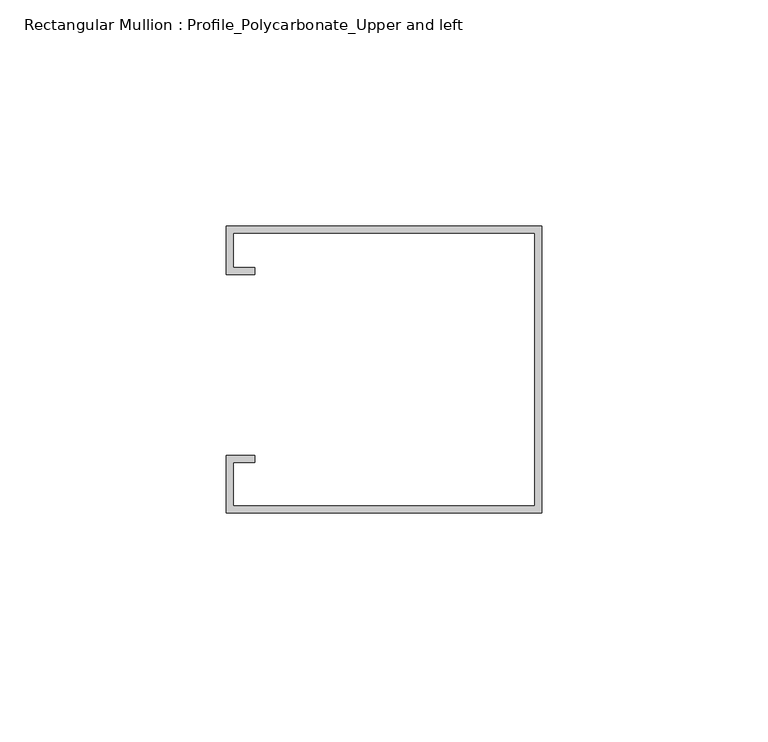
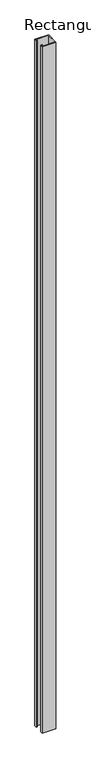
"""IFC4 building model written with IfcOpenShell, lengths in millimetres: member geometry, Rectangular Mullion : Profile_Polycarbonate_Upper and left."""

from ifc_helpers import new_model, si_unit, frame, origin, place, context, project, spatial, polyline, outline, extrude, source, transform, mapped, element, save


def rectangular_mullion_profile_polycarbonate_upper_and_left_4d90c28f(model_context):
    return source(origin(), model_context, "Body", "SweptSolid", [
        extrude(outline(polyline([(0.0, -32.7), (-69.85, -32.7), (-69.85, -20.0), (-63.5, -20.0), (-63.5, -21.5875), (-68.2625, -21.5875), (-68.2625, -31.1125), (-1.5875, -31.1125), (-1.5875, 29.2125), (-68.2625, 29.2125), (-68.2625, 21.5875), (-63.5, 21.5875), (-63.5, 20.0), (-69.85, 20.0), (-69.85, 30.8), (0.0, 30.8), (0.0, -32.7)])), frame((0.0, 0.0, -3695.7), z_axis=(0.0, 0.0, 1.0), x_axis=(1.0, 0.0, 0.0)), (0.0, 0.0, 1.0), 3695.7),
    ])


if __name__ == "__main__":
    model = new_model("IFC4")
    model_context = context("Model", 3, world=origin())
    ifc_project = project(units=[si_unit("LENGTHUNIT", "METRE", prefix="MILLI")], contexts=[model_context])
    site = spatial("IfcSite", under=ifc_project)
    building = spatial("IfcBuilding", under=site)
    placement = place(None, origin())
    rectangular_mullion_profile_polycarbonate_upper_and_left_shape = rectangular_mullion_profile_polycarbonate_upper_and_left_4d90c28f(model_context)
    element("IfcMember", 1, ObjectType="Rectangular Mullion : Profile_Polycarbonate_Upper and left", at=placement, inside=building, context=model_context, shape_type="MappedRepresentation", body=[
        mapped(rectangular_mullion_profile_polycarbonate_upper_and_left_shape, transform((0.0, 0.0, 0.0), x_axis=(1.0, 0.0, 0.0), y_axis=(0.0, 1.0, 0.0), z_axis=(0.0, 0.0, 1.0))),
    ])
    save(model, "model.ifc")

# Revit data of these elements
# Type "Rectangular Mullion : Profile_Polycarbonate_Upper and left"
#   built-in parameter 1007322 = 0.208333 (stored number, unit not read)
#   built-in parameter 1007321 = 0.00520833 (stored number, unit not read)
#   built-in parameter 1007320 = 0 (stored number, unit not read)
